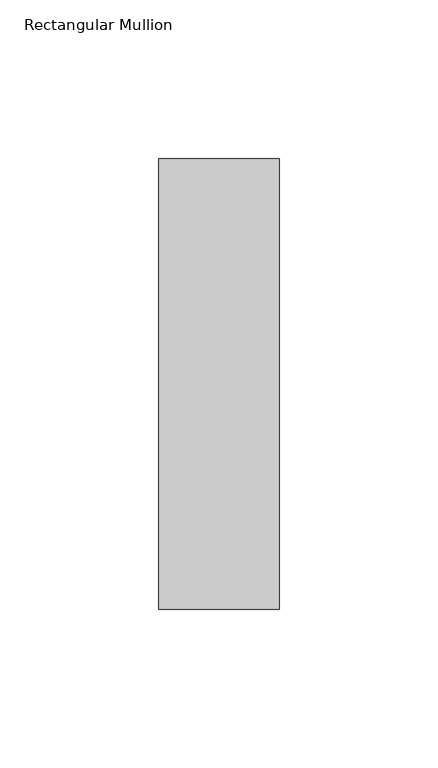
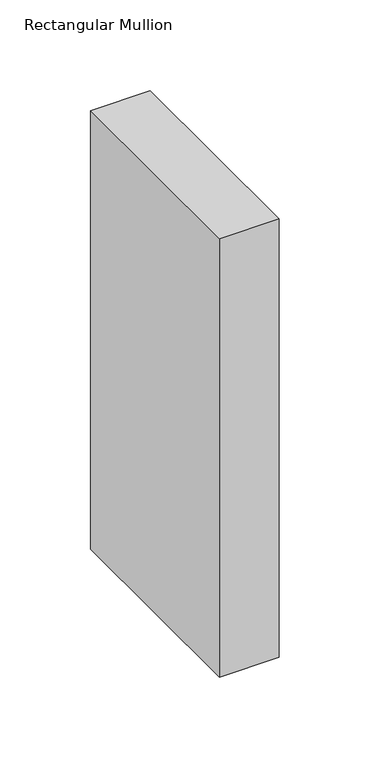
"""IFC4 building model written with IfcOpenShell, lengths in millimetres: member geometry, Rectangular Mullion : NLRS_21_CWM_hsb-regel 38x142_gen_rsf."""

from ifc_helpers import new_model, si_unit, frame, origin, place, context, project, spatial, polyline, outline, extrude, source, transform, mapped, element, save


def rectangular_mullion_c53917db(model_context):
    return source(origin(), model_context, "Body", "SweptSolid", [
        extrude(outline(polyline([(19.0, -71.0), (-19.0, -71.0), (-19.0, 71.0), (19.0, 71.0), (19.0, -71.0)])), frame((0.0, 0.0, -295.0), z_axis=(0.0, 0.0, 1.0), x_axis=(1.0, 0.0, 0.0)), (0.0, 0.0, 1.0), 295.0),
    ])


if __name__ == "__main__":
    model = new_model("IFC4")
    model_context = context("Model", 3, world=origin())
    ifc_project = project(units=[si_unit("LENGTHUNIT", "METRE", prefix="MILLI")], contexts=[model_context])
    site = spatial("IfcSite", under=ifc_project)
    building = spatial("IfcBuilding", under=site)
    placement = place(None, origin())
    rectangular_mullion_shape = rectangular_mullion_c53917db(model_context)
    element("IfcMember", 1, ObjectType="Rectangular Mullion : NLRS_21_CWM_hsb-regel 38x142_gen_rsf", at=placement, inside=building, context=model_context, shape_type="MappedRepresentation", body=[
        mapped(rectangular_mullion_shape, transform((0.0, 0.0, 0.0), x_axis=(1.0, 0.0, 0.0), y_axis=(0.0, 1.0, 0.0), z_axis=(0.0, 0.0, 1.0))),
    ])
    save(model, "model.ifc")

# Revit data of these elements
# Type "Rectangular Mullion : NLRS_21_CWM_hsb-regel 38x142_gen_rsf"
#   Export Type to IFC As = "IfcWall"
#   Type IfcGUID = "07M7mRoiH1CR8m_RSKIwpF"
#   Assembly Code = "21.10"
#   built-in parameter 1007322 = 0.465879 (stored number, unit not read)
#   built-in parameter 1007321 = 0.062336 (stored number, unit not read)
#   built-in parameter 1007320 = 0.062336 (stored number, unit not read)
# Element 1 (IfcMember, "Rectangular Mullion : NLRS_21_CWM_hsb-regel 38x142_gen_rsf")
#   Materials on its faces: "NLRS_i2_hout naaldhout vuren_gen_rsf"
# Materials
#   "NLRS_i2_hout naaldhout vuren_gen_rsf": class "I - Hout", colour RGB 234 199 147, transparency 0, Keynote = "i2", Manufacturer = "Revit Standards Foundation", URL = "www.revitstandards.org", Description = "hout vuren", Cost = 0
